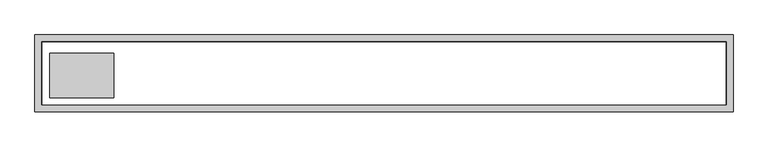
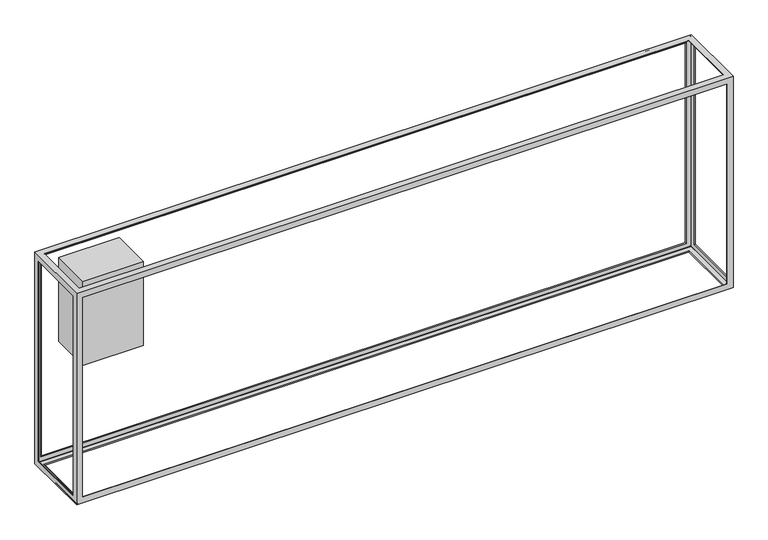
"""IFC4 building model written with IfcOpenShell, lengths in millimetres: beam geometry, Plumbing Bulkhead : EX. BULKHEAD 3 (MODIFIED)."""

from ifc_helpers import new_model, si_unit, frame, origin, place, context, project, spatial, polyline, ellipse_curve, outline, extrude, source, transform, mapped, element, save
from ifc_brep_helpers import plane_surface, cylinder_surface, revolved_surface, advanced_brep


def beam_dc317476(model_context):
    return source(origin(), model_context, "Body", "SolidModel", [
        extrude(outline(polyline([(379.0365927, 279.4), (379.0365927, 66.5145898), (70.4236299, 66.5145898), (70.4236299, 279.4), (379.0365927, 279.4)])), frame((0.0, 0.0, 688.452765), z_axis=(0.0, 0.0, 1.0), x_axis=(1.0, 0.0, 0.0)), (0.0, 0.0, 1.0), 454.547235),
        advanced_brep(
        [(0.0, 0.0, 1143.0), (0.0, 368.3, 1143.0), (0.0, 368.3, 0.0), (0.0, 0.0, 0.0), (0.0, 31.75, 1111.25), (0.0, 31.75, 31.75), (0.0, 336.55, 31.75), (0.0, 336.55, 1111.25), (3352.8, 0.0, 0.0), (3352.8, 368.3, 0.0), (3352.8, 368.3, 1143.0), (3352.8, 0.0, 1143.0), (3352.8, 336.55, 31.75), (3352.8, 31.75, 31.75), (3352.8, 31.75, 1111.25), (3352.8, 336.55, 1111.25), (3321.05, 336.55, 0.0), (31.75, 336.55, 0.0), (31.75, 31.75, 0.0), (3321.05, 31.75, 0.0), (3324.225, 339.725, 3.175), (28.575, 339.725, 3.175), (3348.0375, 4.7625, 3.175), (3348.0375, 363.5375, 3.175), (4.7625, 363.5375, 3.175), (4.7625, 4.7625, 3.175), (3324.225, 28.575, 3.175), (28.575, 28.575, 3.175), (3348.0375, 365.125, 4.7625), (4.7625, 365.125, 4.7625), (3.639968, 364.660032, 3.639968), (3349.160032, 364.660032, 3.639968), (3348.0375, 365.125, 1138.2375), (4.7625, 365.125, 1138.2375), (3324.225, 365.125, 1114.425), (3324.225, 365.125, 28.575), (28.575, 365.125, 28.575), (28.575, 365.125, 1114.425), (3321.05, 368.3, 31.75), (31.75, 368.3, 31.75), (3321.05, 368.3, 1111.25), (31.75, 368.3, 1111.25), (31.75, 31.75, 1143.0), (31.75, 336.55, 1143.0), (3321.05, 336.55, 1143.0), (3321.05, 31.75, 1143.0), (3349.625, 339.725, 28.575), (3349.625, 339.725, 1114.425), (3349.625, 363.5375, 4.7625), (3349.625, 4.7625, 4.7625), (3349.625, 4.7625, 1138.2375), (3349.625, 363.5375, 1138.2375), (3349.625, 28.575, 28.575), (3349.625, 28.575, 1114.425), (3349.160032, 364.660032, 1139.360032), (28.575, 339.725, 1139.825), (3324.225, 339.725, 1139.825), (4.7625, 4.7625, 1139.825), (4.7625, 363.5375, 1139.825), (3348.0375, 363.5375, 1139.825), (3348.0375, 4.7625, 1139.825), (28.575, 28.575, 1139.825), (3324.225, 28.575, 1139.825), (3.639968, 364.660032, 1139.360032), (3.175, 339.725, 1114.425), (3.175, 339.725, 28.575), (3.175, 363.5375, 1138.2375), (3.175, 4.7625, 1138.2375), (3.175, 4.7625, 4.7625), (3.175, 363.5375, 4.7625), (3.175, 28.575, 1114.425), (3.175, 28.575, 28.575), (3321.05, 0.0, 1111.25), (3321.05, 0.0, 31.75), (31.75, 0.0, 31.75), (31.75, 0.0, 1111.25), (3349.160032, 3.639968, 3.639968), (3348.0375, 3.175, 1138.2375), (4.7625, 3.175, 1138.2375), (3.639968, 3.639968, 1139.360032), (3349.160032, 3.639968, 1139.360032), (3348.0375, 3.175, 4.7625), (4.7625, 3.175, 4.7625), (3324.225, 3.175, 28.575), (3324.225, 3.175, 1114.425), (28.575, 3.175, 1114.425), (28.575, 3.175, 28.575), (3.639968, 3.639968, 3.639968)],
        [
            (0, 1),
            (1, 2),
            (2, 3),
            (3, 0),
            (4, 5),
            (5, 6),
            (6, 7),
            (7, 4),
            (8, 9),
            (9, 10),
            (10, 11),
            (11, 8),
            (12, 13),
            (13, 14),
            (14, 15),
            (15, 12),
            (2, 9),
            (8, 3),
            (16, 17),
            (17, 18),
            (18, 19),
            (19, 16),
            (16, 20, ellipse_curve(frame((3324.225, 339.725, 0.0), z_axis=(-0.7071067811865475, 0.7071067811865475, 0.0), x_axis=(-0.7071067811865476, -0.7071067811865474, 0.0)), 4.4901281, 3.175)),
            (20, 21),
            (21, 17, ellipse_curve(frame((28.575, 339.725, 0.0), z_axis=(0.7071067811865454, 0.7071067811865498, 0.0), x_axis=(-0.7071067811865497, 0.7071067811865454, 0.0)), 4.4901281, 3.175)),
            (22, 23),
            (23, 24),
            (24, 25),
            (25, 22),
            (20, 26),
            (26, 27),
            (27, 21),
            (28, 29),
            (29, 30, ellipse_curve(frame((4.7625, 363.5375, 4.7625), z_axis=(-0.7071067811865439, 0.0, 0.7071067811865511), x_axis=(0.7071067811865511, 0.0, 0.7071067811865438)), 2.245064, 1.5875)),
            (30, 24, ellipse_curve(frame((4.7625, 363.5375, 4.7625), z_axis=(-0.7071067811865454, -0.7071067811865498, 0.0), x_axis=(0.7071067811865497, -0.7071067811865454, 0.0)), 2.245064, 1.5875)),
            (23, 31, ellipse_curve(frame((3348.0375, 363.5375, 4.7625), z_axis=(0.7071067811865475, -0.7071067811865475, 0.0), x_axis=(0.7071067811865476, 0.7071067811865474, 0.0)), 2.245064, 1.5875)),
            (31, 28, ellipse_curve(frame((3348.0375, 363.5375, 4.7625), z_axis=(0.7071067811865475, 0.0, 0.7071067811865476), x_axis=(0.7071067811865475, 0.0, -0.7071067811865475)), 2.245064, 1.5875)),
            (28, 32),
            (32, 33),
            (33, 29),
            (34, 35),
            (35, 36),
            (36, 37),
            (37, 34),
            (35, 38, ellipse_curve(frame((3324.225, 368.3, 28.575), z_axis=(-0.7071067811865475, 0.0, -0.7071067811865476), x_axis=(-0.7071067811865475, 0.0, 0.7071067811865475)), 4.4901281, 3.175)),
            (38, 39),
            (39, 36, ellipse_curve(frame((28.575, 368.3, 28.575), z_axis=(0.7071067811865439, 0.0, -0.7071067811865511), x_axis=(-0.7071067811865511, 0.0, -0.7071067811865438)), 4.4901281, 3.175)),
            (1, 10),
            (38, 40),
            (40, 41),
            (41, 39),
            (0, 11),
            (42, 43),
            (43, 44),
            (44, 45),
            (45, 42),
            (46, 12, ellipse_curve(frame((3352.8, 339.725, 28.575), z_axis=(0.0, 0.7071067811865429, 0.7071067811865522), x_axis=(0.0, 0.7071067811865523, -0.7071067811865427)), 4.4901281, 3.175)),
            (15, 47, ellipse_curve(frame((3352.8, 339.725, 1114.425), z_axis=(0.0, 0.707106781186551, -0.7071067811865441), x_axis=(0.0, -0.7071067811865441, -0.7071067811865509)), 4.4901281, 3.175)),
            (47, 46),
            (48, 49),
            (49, 50),
            (50, 51),
            (51, 48),
            (52, 46),
            (47, 53),
            (53, 52),
            (31, 48, ellipse_curve(frame((3348.0375, 363.5375, 4.7625), z_axis=(0.0, -0.7071067811865429, -0.7071067811865522), x_axis=(0.0, -0.7071067811865523, 0.7071067811865427)), 2.245064, 1.5875)),
            (51, 54, ellipse_curve(frame((3348.0375, 363.5375, 1138.2375), z_axis=(0.0, -0.707106781186551, 0.7071067811865441), x_axis=(0.0, 0.7071067811865441, 0.7071067811865509)), 2.245064, 1.5875)),
            (54, 32, ellipse_curve(frame((3348.0375, 363.5375, 1138.2375), z_axis=(-0.7071067811865475, 0.0, 0.7071067811865475), x_axis=(0.7071067811865474, 0.0, 0.7071067811865476)), 2.245064, 1.5875)),
            (34, 40, ellipse_curve(frame((3324.225, 368.3, 1114.425), z_axis=(0.7071067811865475, 0.0, -0.7071067811865475), x_axis=(-0.7071067811865474, 0.0, -0.7071067811865476)), 4.4901281, 3.175)),
            (43, 55, ellipse_curve(frame((28.575, 339.725, 1143.0), z_axis=(0.707106781186548, 0.7071067811865469, 0.0), x_axis=(-0.707106781186547, 0.7071067811865478, 0.0)), 4.4901281, 3.175)),
            (55, 56),
            (56, 44, ellipse_curve(frame((3324.225, 339.725, 1143.0), z_axis=(-0.7071067811865469, 0.707106781186548, 0.0), x_axis=(-0.7071067811865481, -0.7071067811865468, 0.0)), 4.4901281, 3.175)),
            (57, 58),
            (58, 59),
            (59, 60),
            (60, 57),
            (55, 61),
            (61, 62),
            (62, 56),
            (54, 59, ellipse_curve(frame((3348.0375, 363.5375, 1138.2375), z_axis=(0.7071067811865469, -0.707106781186548, 0.0), x_axis=(0.7071067811865481, 0.7071067811865468, 0.0)), 2.245064, 1.5875)),
            (58, 63, ellipse_curve(frame((4.7625, 363.5375, 1138.2375), z_axis=(-0.707106781186548, -0.7071067811865469, 0.0), x_axis=(0.707106781186547, -0.7071067811865478, 0.0)), 2.245064, 1.5875)),
            (63, 33, ellipse_curve(frame((4.7625, 363.5375, 1138.2375), z_axis=(-0.7071067811865511, 0.0, -0.7071067811865439), x_axis=(0.7071067811865439, 0.0, -0.7071067811865511)), 2.245064, 1.5875)),
            (37, 41, ellipse_curve(frame((28.575, 368.3, 1114.425), z_axis=(0.7071067811865511, 0.0, 0.7071067811865439), x_axis=(-0.7071067811865439, 0.0, 0.7071067811865511)), 4.4901281, 3.175)),
            (64, 7, ellipse_curve(frame((0.0, 339.725, 1114.425), z_axis=(0.0, 0.7071067811865487, -0.7071067811865462), x_axis=(0.0, -0.7071067811865462, -0.7071067811865489)), 4.4901281, 3.175)),
            (6, 65, ellipse_curve(frame((0.0, 339.725, 28.575), z_axis=(0.0, 0.707106781186545, 0.70710678118655), x_axis=(0.0, 0.7071067811865499, -0.707106781186545)), 4.4901281, 3.175)),
            (65, 64),
            (66, 67),
            (67, 68),
            (68, 69),
            (69, 66),
            (70, 64),
            (65, 71),
            (71, 70),
            (63, 66, ellipse_curve(frame((4.7625, 363.5375, 1138.2375), z_axis=(0.0, -0.7071067811865487, 0.7071067811865462), x_axis=(0.0, 0.7071067811865462, 0.7071067811865489)), 2.245064, 1.5875)),
            (69, 30, ellipse_curve(frame((4.7625, 363.5375, 4.7625), z_axis=(0.0, -0.707106781186545, -0.70710678118655), x_axis=(0.0, -0.7071067811865499, 0.707106781186545)), 2.245064, 1.5875)),
            (72, 73),
            (73, 74),
            (74, 75),
            (75, 72),
            (19, 26, ellipse_curve(frame((3324.225, 28.575, 0.0), z_axis=(0.7071067811865475, 0.7071067811865475, 0.0), x_axis=(0.7071067811865474, -0.7071067811865476, 0.0)), 4.4901281, 3.175)),
            (22, 76, ellipse_curve(frame((3348.0375, 4.7625, 4.7625), z_axis=(-0.7071067811865475, -0.7071067811865475, 0.0), x_axis=(-0.7071067811865474, 0.7071067811865476, 0.0)), 2.245064, 1.5875)),
            (76, 49, ellipse_curve(frame((3348.0375, 4.7625, 4.7625), z_axis=(0.0, -0.7071067811865499, 0.7071067811865451), x_axis=(0.0, 0.7071067811865451, 0.70710678118655)), 2.245064, 1.5875)),
            (52, 13, ellipse_curve(frame((3352.8, 28.575, 28.575), z_axis=(0.0, 0.7071067811865499, -0.7071067811865451), x_axis=(0.0, -0.7071067811865451, -0.70710678118655)), 4.4901281, 3.175)),
            (61, 42, ellipse_curve(frame((28.575, 28.575, 1143.0), z_axis=(0.7071067811865469, -0.707106781186548, 0.0), x_axis=(-0.7071067811865481, -0.7071067811865468, 0.0)), 4.4901281, 3.175)),
            (45, 62, ellipse_curve(frame((3324.225, 28.575, 1143.0), z_axis=(-0.707106781186548, -0.7071067811865469, 0.0), x_axis=(-0.707106781186547, 0.7071067811865478, 0.0)), 4.4901281, 3.175)),
            (77, 78),
            (78, 79, ellipse_curve(frame((4.7625, 4.7625, 1138.2375), z_axis=(-0.7071067811865511, 0.0, -0.7071067811865439), x_axis=(0.7071067811865439, 0.0, -0.7071067811865511)), 2.245064, 1.5875)),
            (79, 57, ellipse_curve(frame((4.7625, 4.7625, 1138.2375), z_axis=(-0.7071067811865469, 0.707106781186548, 0.0), x_axis=(0.7071067811865481, 0.7071067811865468, 0.0)), 2.245064, 1.5875)),
            (60, 80, ellipse_curve(frame((3348.0375, 4.7625, 1138.2375), z_axis=(0.707106781186548, 0.7071067811865469, 0.0), x_axis=(0.707106781186547, -0.7071067811865478, 0.0)), 2.245064, 1.5875)),
            (80, 77, ellipse_curve(frame((3348.0375, 4.7625, 1138.2375), z_axis=(0.7071067811865475, 0.0, -0.7071067811865475), x_axis=(0.7071067811865476, 0.0, 0.7071067811865474)), 2.245064, 1.5875)),
            (77, 81),
            (81, 82),
            (82, 78),
            (83, 84),
            (84, 85),
            (85, 86),
            (86, 83),
            (84, 72, ellipse_curve(frame((3324.225, 0.0, 1114.425), z_axis=(-0.7071067811865475, 0.0, 0.7071067811865475), x_axis=(-0.7071067811865476, 0.0, -0.7071067811865474)), 4.4901281, 3.175)),
            (75, 85, ellipse_curve(frame((28.575, 0.0, 1114.425), z_axis=(0.7071067811865511, 0.0, 0.7071067811865439), x_axis=(-0.7071067811865439, 0.0, 0.7071067811865511)), 4.4901281, 3.175)),
            (18, 27, ellipse_curve(frame((28.575, 28.575, 0.0), z_axis=(0.7071067811865498, -0.7071067811865452, 0.0), x_axis=(-0.7071067811865452, -0.7071067811865498, 0.0)), 4.4901281, 3.175)),
            (25, 87, ellipse_curve(frame((4.7625, 4.7625, 4.7625), z_axis=(-0.7071067811865498, 0.7071067811865452, 0.0), x_axis=(0.7071067811865452, 0.7071067811865498, 0.0)), 2.245064, 1.5875)),
            (87, 82, ellipse_curve(frame((4.7625, 4.7625, 4.7625), z_axis=(-0.7071067811865439, 0.0, 0.7071067811865511), x_axis=(0.7071067811865511, 0.0, 0.7071067811865438)), 2.245064, 1.5875)),
            (81, 76, ellipse_curve(frame((3348.0375, 4.7625, 4.7625), z_axis=(0.7071067811865475, 0.0, 0.7071067811865476), x_axis=(0.7071067811865475, 0.0, -0.7071067811865475)), 2.245064, 1.5875)),
            (73, 83, ellipse_curve(frame((3324.225, 0.0, 28.575), z_axis=(-0.7071067811865475, 0.0, -0.7071067811865476), x_axis=(-0.7071067811865475, 0.0, 0.7071067811865475)), 4.4901281, 3.175)),
            (86, 74, ellipse_curve(frame((28.575, 0.0, 28.575), z_axis=(0.7071067811865439, 0.0, -0.7071067811865511), x_axis=(-0.7071067811865511, 0.0, -0.7071067811865438)), 4.4901281, 3.175)),
            (53, 14, ellipse_curve(frame((3352.8, 28.575, 1114.425), z_axis=(0.0, -0.7071067811865464, -0.7071067811865487), x_axis=(0.0, 0.7071067811865487, -0.7071067811865464)), 4.4901281, 3.175)),
            (80, 50, ellipse_curve(frame((3348.0375, 4.7625, 1138.2375), z_axis=(0.0, 0.7071067811865464, 0.7071067811865487), x_axis=(0.0, -0.7071067811865487, 0.7071067811865464)), 2.245064, 1.5875)),
            (4, 70, ellipse_curve(frame((0.0, 28.575, 1114.425), z_axis=(0.0, -0.7071067811865464, -0.7071067811865487), x_axis=(0.0, 0.7071067811865487, -0.7071067811865464)), 4.4901281, 3.175)),
            (71, 5, ellipse_curve(frame((0.0, 28.575, 28.575), z_axis=(0.0, -0.7071067811865499, 0.7071067811865451), x_axis=(0.0, -0.7071067811865451, -0.7071067811865498)), 4.4901281, 3.175)),
            (87, 68, ellipse_curve(frame((4.7625, 4.7625, 4.7625), z_axis=(0.0, 0.7071067811865499, -0.7071067811865451), x_axis=(0.0, 0.7071067811865451, 0.7071067811865498)), 2.245064, 1.5875)),
            (67, 79, ellipse_curve(frame((4.7625, 4.7625, 1138.2375), z_axis=(0.0, 0.7071067811865464, 0.7071067811865487), x_axis=(0.0, -0.7071067811865487, 0.7071067811865464)), 2.245064, 1.5875)),
        ],
        [
            plane_surface(frame((0.0, 368.3, 0.0), z_axis=(-1.0, 0.0, 0.0), x_axis=(0.0, 0.0, 1.0))),
            plane_surface(frame((3352.8, 368.3, 0.0), z_axis=(1.0, 0.0, 0.0), x_axis=(0.0, 0.0, 1.0))),
            plane_surface(frame((0.0, 368.3, 0.0), z_axis=(0.0, 0.0, -1.0), x_axis=(1.0, 0.0, 0.0))),
            cylinder_surface(frame((0.0, 339.725, 0.0), z_axis=(-1.0, 0.0, 0.0), x_axis=(0.0, -1.0, 0.0)), 3.175),
            plane_surface(frame((0.0, 339.725, 3.175), z_axis=(0.0, 0.0, 1.0), x_axis=(1.0, 0.0, 0.0))),
            revolved_surface(polyline([(3349.6249999785978, 361.95000000000005, 4.7625), (3.175000021402197, 361.95000000000005, 4.7625)]), (0.0, 363.5375, 4.7625), (1.0, 0.0, 0.0)),
            plane_surface(frame((0.0, 365.125, 4.7625), z_axis=(0.0, -1.0, 0.0), x_axis=(1.0, 0.0, 0.0))),
            cylinder_surface(frame((0.0, 368.3, 28.575), z_axis=(-1.0, 0.0, 0.0), x_axis=(0.0, -1.0, 0.0)), 3.175),
            plane_surface(frame((0.0, 368.3, 31.75), z_axis=(0.0, 1.0, 0.0), x_axis=(1.0, 0.0, 0.0))),
            plane_surface(frame((3352.8, 368.3, 1143.0), z_axis=(0.0, 0.0, 1.0), x_axis=(1.0, 0.0, 0.0))),
            cylinder_surface(frame((3352.8, 339.725, 0.0), z_axis=(0.0, 0.0, -1.0), x_axis=(0.0, -1.0, 0.0)), 3.175),
            plane_surface(frame((3349.625, 339.725, 0.0), z_axis=(-1.0, 0.0, 0.0), x_axis=(0.0, 0.0, 1.0))),
            revolved_surface(polyline([(3348.0375, 361.95000000000005, 1139.8249999785978), (3348.0375, 361.95000000000005, 3.175000021402205)]), (3348.0375, 363.5375, 0.0), (0.0, 0.0, 1.0)),
            cylinder_surface(frame((3324.225, 368.3, 0.0), z_axis=(0.0, 0.0, -1.0), x_axis=(0.0, -1.0, 0.0)), 3.175),
            cylinder_surface(frame((0.0, 339.725, 1143.0), z_axis=(-1.0, 0.0, 0.0), x_axis=(0.0, -1.0, 0.0)), 3.175),
            plane_surface(frame((0.0, 363.5375, 1139.825), z_axis=(0.0, 0.0, -1.0), x_axis=(1.0, 0.0, 0.0))),
            revolved_surface(polyline([(3349.6249999785978, 361.95000000000005, 1138.2375), (3.175000021402206, 361.95000000000005, 1138.2375)]), (0.0, 363.5375, 1138.2375), (1.0, 0.0, 0.0)),
            cylinder_surface(frame((0.0, 368.3, 1114.425), z_axis=(-1.0, 0.0, 0.0), x_axis=(0.0, -1.0, 0.0)), 3.175),
            cylinder_surface(frame((0.0, 339.725, 0.0), z_axis=(0.0, 0.0, -1.0), x_axis=(0.0, -1.0, 0.0)), 3.175),
            plane_surface(frame((3.175, 363.5375, 0.0), z_axis=(1.0, 0.0, 0.0), x_axis=(0.0, 0.0, 1.0))),
            revolved_surface(polyline([(4.7625, 361.95000000000005, 1139.8249999785978), (4.7625, 361.95000000000005, 3.1750000214022105)]), (4.7625, 363.5375, 0.0), (0.0, 0.0, 1.0)),
            cylinder_surface(frame((28.575, 368.3, 0.0), z_axis=(0.0, 0.0, -1.0), x_axis=(0.0, -1.0, 0.0)), 3.175),
            plane_surface(frame((3352.8, 0.0, 0.0), z_axis=(0.0, -1.0, 0.0), x_axis=(0.0, 0.0, 1.0))),
            cylinder_surface(frame((3324.225, 0.0, 0.0), z_axis=(0.0, -1.0, 0.0), x_axis=(-1.0, 0.0, 0.0)), 3.175),
            revolved_surface(polyline([(3346.45, 365.1249999785978, 4.7625), (3346.45, 3.1750000214022047, 4.7625)]), (3348.0375, 0.0, 4.7625), (0.0, 1.0, 0.0)),
            cylinder_surface(frame((3352.8, 0.0, 28.575), z_axis=(0.0, -1.0, 0.0), x_axis=(-1.0, 0.0, 0.0)), 3.175),
            cylinder_surface(frame((0.0, 28.575, 1143.0), z_axis=(-1.0, 0.0, 0.0), x_axis=(0.0, 1.0, 0.0)), 3.175),
            revolved_surface(polyline([(3349.6249999785978, 6.35, 1138.2375), (3.1750000214022034, 6.35, 1138.2375)]), (0.0, 4.7625, 1138.2375), (1.0, 0.0, 0.0)),
            plane_surface(frame((0.0, 3.175, 1138.2375), z_axis=(0.0, 1.0, 0.0), x_axis=(1.0, 0.0, 0.0))),
            cylinder_surface(frame((0.0, 0.0, 1114.425), z_axis=(-1.0, 0.0, 0.0), x_axis=(0.0, 1.0, 0.0)), 3.175),
            cylinder_surface(frame((0.0, 28.575, 0.0), z_axis=(-1.0, 0.0, 0.0), x_axis=(0.0, 1.0, 0.0)), 3.175),
            revolved_surface(polyline([(3349.6249999785978, 6.35, 4.7625), (3.175000021402197, 6.35, 4.7625)]), (0.0, 4.7625, 4.7625), (1.0, 0.0, 0.0)),
            cylinder_surface(frame((0.0, 0.0, 28.575), z_axis=(-1.0, 0.0, 0.0), x_axis=(0.0, 1.0, 0.0)), 3.175),
            cylinder_surface(frame((3352.8, 28.575, 0.0), z_axis=(0.0, 0.0, -1.0), x_axis=(0.0, 1.0, 0.0)), 3.175),
            revolved_surface(polyline([(3348.0375, 6.35, 1139.8249999785978), (3348.0375, 6.35, 3.1750000214021994)]), (3348.0375, 4.7625, 0.0), (0.0, 0.0, 1.0)),
            cylinder_surface(frame((3324.225, 0.0, 0.0), z_axis=(0.0, 0.0, -1.0), x_axis=(0.0, 1.0, 0.0)), 3.175),
            cylinder_surface(frame((0.0, 28.575, 0.0), z_axis=(0.0, 0.0, -1.0), x_axis=(0.0, 1.0, 0.0)), 3.175),
            revolved_surface(polyline([(4.7625, 6.35, 1139.8249999785978), (4.7625, 6.35, 3.1750000214022)]), (4.7625, 4.7625, 0.0), (0.0, 0.0, 1.0)),
            cylinder_surface(frame((28.575, 0.0, 0.0), z_axis=(0.0, 0.0, -1.0), x_axis=(0.0, 1.0, 0.0)), 3.175),
            cylinder_surface(frame((28.575, 0.0, 1143.0), z_axis=(0.0, -1.0, 0.0), x_axis=(1.0, 0.0, 0.0)), 3.175),
            revolved_surface(polyline([(6.35, 365.1249999785978, 1138.2375), (6.35, 3.1750000214022025, 1138.2375)]), (4.7625, 0.0, 1138.2375), (0.0, 1.0, 0.0)),
            cylinder_surface(frame((0.0, 0.0, 1114.425), z_axis=(0.0, -1.0, 0.0), x_axis=(1.0, 0.0, 0.0)), 3.175),
            cylinder_surface(frame((3324.225, 0.0, 1143.0), z_axis=(0.0, -1.0, 0.0), x_axis=(-1.0, 0.0, 0.0)), 3.175),
            revolved_surface(polyline([(3346.45, 365.1249999785978, 1138.2375), (3346.45, 3.1750000214022025, 1138.2375)]), (3348.0375, 0.0, 1138.2375), (0.0, 1.0, 0.0)),
            cylinder_surface(frame((3352.8, 0.0, 1114.425), z_axis=(0.0, -1.0, 0.0), x_axis=(-1.0, 0.0, 0.0)), 3.175),
            cylinder_surface(frame((28.575, 0.0, 0.0), z_axis=(0.0, -1.0, 0.0), x_axis=(1.0, 0.0, 0.0)), 3.175),
            revolved_surface(polyline([(6.35, 365.1249999785978, 4.7625), (6.35, 3.1750000214022, 4.7625)]), (4.7625, 0.0, 4.7625), (0.0, 1.0, 0.0)),
            cylinder_surface(frame((0.0, 0.0, 28.575), z_axis=(0.0, -1.0, 0.0), x_axis=(1.0, 0.0, 0.0)), 3.175),
        ],
        [
            (0, [[1, 2, 3, 4], [5, 6, 7, 8]]),
            (1, [[9, 10, 11, 12], [13, 14, 15, 16]]),
            (2, [[-3, 17, -9, 18], [19, 20, 21, 22]]),
            (3, [[23, 24, 25, -19]]),
            (4, [[26, 27, 28, 29], [30, 31, 32, -24]]),
            (5, [[33, 34, 35, -27, 36, 37]]),
            (6, [[38, 39, 40, -33], [41, 42, 43, 44]]),
            (7, [[45, 46, 47, -42]]),
            (8, [[-10, -17, -2, 48], [49, 50, 51, -46]]),
            (9, [[-1, 52, -11, -48], [53, 54, 55, 56]]),
            (10, [[57, -16, 58, 59]]),
            (11, [[60, 61, 62, 63], [64, -59, 65, 66]]),
            (12, [[-38, -37, 67, -63, 68, 69]]),
            (13, [[-45, -41, 70, -49]]),
            (14, [[71, 72, 73, -54]]),
            (15, [[74, 75, 76, 77], [78, 79, 80, -72]]),
            (16, [[-39, -69, 81, -75, 82, 83]]),
            (17, [[-70, -44, 84, -50]]),
            (18, [[85, -7, 86, 87]]),
            (19, [[88, 89, 90, 91], [92, -87, 93, 94]]),
            (20, [[-40, -83, 95, -91, 96, -34]]),
            (21, [[-43, -47, -51, -84]]),
            (22, [[-18, -12, -52, -4], [97, 98, 99, 100]]),
            (23, [[-23, -22, 101, -30]]),
            (24, [[-36, -26, 102, 103, -60, -67]]),
            (25, [[-57, -64, 104, -13]]),
            (26, [[105, -56, 106, -79]]),
            (27, [[107, 108, 109, -77, 110, 111]]),
            (28, [[112, 113, 114, -107], [115, 116, 117, 118]]),
            (29, [[119, -100, 120, -116]]),
            (30, [[-101, -21, 121, -31]]),
            (31, [[-102, -29, 122, 123, -113, 124]]),
            (32, [[125, -118, 126, -98]]),
            (33, [[-104, -66, 127, -14]]),
            (34, [[-103, -124, -112, -111, 128, -61]]),
            (35, [[-115, -125, -97, -119]]),
            (36, [[129, -94, 130, -5]]),
            (37, [[-114, -123, 131, -89, 132, -108]]),
            (38, [[-117, -120, -99, -126]]),
            (39, [[-53, -105, -78, -71]]),
            (40, [[-82, -74, -109, -132, -88, -95]]),
            (41, [[-8, -85, -92, -129]]),
            (42, [[-80, -106, -55, -73]]),
            (43, [[-68, -62, -128, -110, -76, -81]]),
            (44, [[-15, -127, -65, -58]]),
            (45, [[-20, -25, -32, -121]]),
            (46, [[-90, -131, -122, -28, -35, -96]]),
            (47, [[-93, -86, -6, -130]]),
        ],
    ),
    ])


if __name__ == "__main__":
    model = new_model("IFC4")
    model_context = context("Model", 3, world=origin())
    ifc_project = project(units=[si_unit("LENGTHUNIT", "METRE", prefix="MILLI")], contexts=[model_context])
    site = spatial("IfcSite", under=ifc_project)
    building = spatial("IfcBuilding", under=site)
    placement = place(None, origin())
    beam_shape = beam_dc317476(model_context)
    element("IfcBeam", 1, ObjectType="Plumbing Bulkhead : EX. BULKHEAD 3 (MODIFIED)", at=placement, inside=building, context=model_context, shape_type="MappedRepresentation", body=[
        mapped(beam_shape, transform((0.0, 0.0, 0.0), x_axis=(1.0, 0.0, 0.0), y_axis=(0.0, 1.0, 0.0), z_axis=(0.0, 0.0, 1.0))),
    ])
    save(model, "model.ifc")

# Revit data of these elements
# Type "Plumbing Bulkhead : EX. BULKHEAD 3 (MODIFIED)"
#   Length = 11' - 0"
#   Height = 3' - 9"
#   Depth = 1' - 2 1/2"
#   EP MATERIAL = ELECTRICAL PANEL
#   Structural Material = none
# Element 1 (IfcBeam, "Plumbing Bulkhead : EX. BULKHEAD 3 (MODIFIED)")
#   Materials on its faces: "ELECTRICAL PANEL"
# Materials
#   "ELECTRICAL PANEL": class "Generic", colour RGB 255 255 255, transparency 0, Cost = 0
